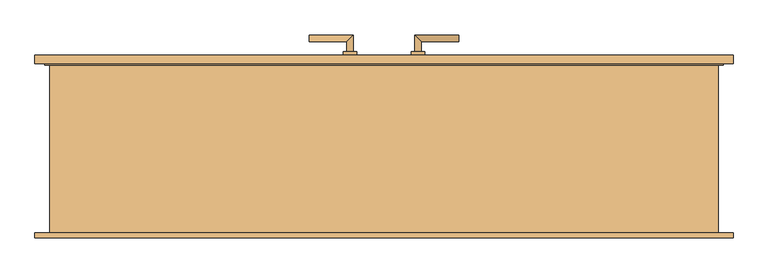
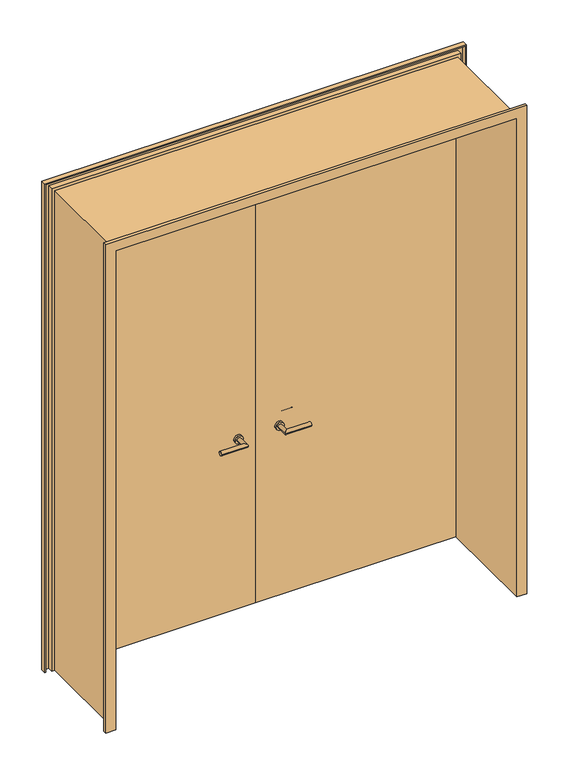
"""IFC4 building model written with IfcOpenShell, lengths in millimetres: door geometry, Drehflügel 2-flg - Variabel : Drehflügel 2-flg - Variabel."""

from ifc_helpers import new_model, si_unit, point, frame, frame_2d, origin, place, context, project, spatial, polyline, circle_curve, ellipse_curve, trimmed, segment, composite_curve, outline, extrude, faceted_brep, source, transform, mapped, element, save
from ifc_brep_helpers import plane_surface, cylinder_surface, advanced_brep


def door_c7457bb2(model_context):
    return source(origin(), model_context, "Body", "SolidModel", [
        advanced_brep(
        [(-90.0, 239.4346141, 1000.0), (-110.0, 239.4346141, 1000.0), (-110.0, 189.4346141, 1000.0), (-90.0, 169.4346141, 1000.0), (-220.0, 169.4346141, 1000.0), (-220.0, 189.4346141, 1000.0)],
        [
            (0, 1, circle_curve(frame((-100.0, 239.4346141, 1000.0), z_axis=(0.0, 1.0, 0.0), x_axis=(-1.0, 0.0, 0.0)), 10.0)),
            (1, 0, circle_curve(frame((-100.0, 239.4346141, 1000.0), z_axis=(0.0, 1.0, 0.0), x_axis=(-1.0, 0.0, 0.0)), 10.0)),
            (1, 2),
            (2, 3, ellipse_curve(frame((-100.0, 179.4346141, 1000.0), z_axis=(0.7071067811865385, 0.7071067811865565, 0.0), x_axis=(-0.7071067811865563, 0.7071067811865386, 0.0)), 14.1421356, 10.0)),
            (3, 0),
            (3, 2, ellipse_curve(frame((-100.0, 179.4346141, 1000.0), z_axis=(0.7071067811865385, 0.7071067811865565, 0.0), x_axis=(-0.7071067811865563, 0.7071067811865386, 0.0)), 14.1421356, 10.0)),
            (4, 5, circle_curve(frame((-220.0, 179.4346141, 1000.0), z_axis=(-1.0, 0.0, 0.0), x_axis=(0.0, 1.0, 0.0)), 10.0)),
            (5, 4, circle_curve(frame((-220.0, 179.4346141, 1000.0), z_axis=(-1.0, 0.0, 0.0), x_axis=(0.0, 1.0, 0.0)), 10.0)),
            (2, 5),
            (4, 3),
        ],
        [
            plane_surface(frame((-100.0, 239.4346141, -287.7526403), z_axis=(0.0, 1.0, 0.0), x_axis=(0.0, 0.0, 1.0))),
            cylinder_surface(frame((-100.0, 239.4346141, 1000.0), z_axis=(0.0, 1.0, 0.0), x_axis=(-1.0, 0.0, 0.0)), 10.0),
            plane_surface(frame((-220.0, 179.4346141, -287.7526403), z_axis=(-1.0, 0.0, 0.0), x_axis=(0.0, 0.0, 1.0))),
            cylinder_surface(frame((-100.0, 179.4346141, 1000.0), z_axis=(1.0, 0.0, 0.0), x_axis=(0.0, 1.0, 0.0)), 10.0),
        ],
        [
            (0, [[1, 2]]),
            (1, [[3, 4, 5, -2]]),
            (1, [[-5, 6, -3, -1]]),
            (2, [[7, 8]]),
            (3, [[9, -7, 10, -4]]),
            (3, [[-10, -8, -9, -6]]),
        ],
    ),
        advanced_brep(
        [(-110.0, 299.4346141, 1000.0), (-90.0, 299.4346141, 1000.0), (-90.0, 349.4346141, 1000.0), (-110.0, 329.4346141, 1000.0), (-220.0, 329.4346141, 1000.0), (-220.0, 349.4346141, 1000.0)],
        [
            (0, 1, circle_curve(frame((-100.0, 299.4346141, 1000.0), z_axis=(0.0, -1.0, 0.0), x_axis=(1.0, 0.0, 0.0)), 10.0)),
            (1, 0, circle_curve(frame((-100.0, 299.4346141, 1000.0), z_axis=(0.0, -1.0, 0.0), x_axis=(1.0, 0.0, 0.0)), 10.0)),
            (1, 2),
            (2, 3, ellipse_curve(frame((-100.0, 339.4346141, 1000.0), z_axis=(0.7071067811865475, -0.7071067811865475, 0.0), x_axis=(-0.7071067811865474, -0.7071067811865476, 0.0)), 14.1421356, 10.0)),
            (3, 0),
            (3, 2, ellipse_curve(frame((-100.0, 339.4346141, 1000.0), z_axis=(0.7071067811865475, -0.7071067811865475, 0.0), x_axis=(-0.7071067811865474, -0.7071067811865476, 0.0)), 14.1421356, 10.0)),
            (4, 5, circle_curve(frame((-220.0, 339.4346141, 1000.0), z_axis=(-1.0, 0.0, 0.0), x_axis=(0.0, 1.0, 0.0)), 10.0)),
            (5, 4, circle_curve(frame((-220.0, 339.4346141, 1000.0), z_axis=(-1.0, 0.0, 0.0), x_axis=(0.0, 1.0, 0.0)), 10.0)),
            (2, 5),
            (4, 3),
        ],
        [
            plane_surface(frame((-100.0, 299.4346141, -287.7526403), z_axis=(0.0, -1.0, 0.0), x_axis=(0.0, 0.0, 1.0))),
            cylinder_surface(frame((-100.0, 299.4346141, 1000.0), z_axis=(0.0, -1.0, 0.0), x_axis=(1.0, 0.0, 0.0)), 10.0),
            plane_surface(frame((-220.0, 339.4346141, -287.7526403), z_axis=(-1.0, 0.0, 0.0), x_axis=(0.0, 0.0, 1.0))),
            cylinder_surface(frame((-100.0, 339.4346141, 1000.0), z_axis=(1.0, 0.0, 0.0), x_axis=(0.0, 1.0, 0.0)), 10.0),
        ],
        [
            (0, [[1, 2]]),
            (1, [[3, 4, 5, -2]]),
            (1, [[-5, 6, -3, -1]]),
            (2, [[7, 8]]),
            (3, [[9, -7, 10, -4]]),
            (3, [[-10, -8, -9, -6]]),
        ],
    ),
        extrude(outline(composite_curve([segment(trimmed(circle_curve(frame_2d((1000.0, -100.0)), 20.0), [point((1000.0, -80.0))], [point((1000.0, -120.0))], False, "CARTESIAN"), True, "CONTINUOUS"), segment(trimmed(circle_curve(frame_2d((1000.0, -100.0)), 20.0), [point((1000.0, -120.0))], [point((1000.0, -80.0))], False, "CARTESIAN"), True, "CONTINUOUS")], self_intersect=False)), frame((0.0, 229.4346141, 0.0), z_axis=(0.0, 1.0, 0.0), x_axis=(0.0, 0.0, 1.0)), (0.0, 0.0, 1.0), 10.0),
        extrude(outline(composite_curve([segment(trimmed(circle_curve(frame_2d((1000.0, -100.0)), 20.0), [point((1000.0, -80.0))], [point((1000.0, -120.0))], False, "CARTESIAN"), True, "CONTINUOUS"), segment(trimmed(circle_curve(frame_2d((1000.0, -100.0)), 20.0), [point((1000.0, -120.0))], [point((1000.0, -80.0))], False, "CARTESIAN"), True, "CONTINUOUS")], self_intersect=False)), frame((0.0, 289.4346141, 0.0), z_axis=(0.0, 1.0, 0.0), x_axis=(0.0, 0.0, 1.0)), (0.0, 0.0, 1.0), 10.0),
        advanced_brep(
        [(90.0, 239.4346141, 1000.0), (110.0, 239.4346141, 1000.0), (90.0, 169.4346141, 1000.0), (110.0, 189.4346141, 1000.0), (220.0, 169.4346141, 1000.0), (220.0, 189.4346141, 1000.0)],
        [
            (0, 1, circle_curve(frame((100.0, 239.4346141, 1000.0), z_axis=(0.0, 1.0, 0.0), x_axis=(1.0, 0.0, 0.0)), 10.0)),
            (1, 0, circle_curve(frame((100.0, 239.4346141, 1000.0), z_axis=(0.0, 1.0, 0.0), x_axis=(1.0, 0.0, 0.0)), 10.0)),
            (0, 2),
            (2, 3, ellipse_curve(frame((100.0, 179.4346141, 1000.0), z_axis=(-0.7071067811865385, 0.7071067811865565, 0.0), x_axis=(0.7071067811865563, 0.7071067811865386, 0.0)), 14.1421356, 10.0)),
            (3, 1),
            (3, 2, ellipse_curve(frame((100.0, 179.4346141, 1000.0), z_axis=(-0.7071067811865385, 0.7071067811865565, 0.0), x_axis=(0.7071067811865563, 0.7071067811865386, 0.0)), 14.1421356, 10.0)),
            (4, 5, circle_curve(frame((220.0, 179.4346141, 1000.0), z_axis=(1.0, 0.0, 0.0), x_axis=(0.0, 1.0, 0.0)), 10.0)),
            (5, 4, circle_curve(frame((220.0, 179.4346141, 1000.0), z_axis=(1.0, 0.0, 0.0), x_axis=(0.0, 1.0, 0.0)), 10.0)),
            (2, 4),
            (5, 3),
        ],
        [
            plane_surface(frame((100.0, 239.4346141, -287.7526403), z_axis=(0.0, 1.0, 0.0), x_axis=(0.0, 0.0, 1.0))),
            cylinder_surface(frame((100.0, 239.4346141, 1000.0), z_axis=(0.0, 1.0, 0.0), x_axis=(1.0, 0.0, 0.0)), 10.0),
            plane_surface(frame((220.0, 179.4346141, -287.7526403), z_axis=(1.0, 0.0, 0.0), x_axis=(0.0, 0.0, 1.0))),
            cylinder_surface(frame((100.0, 179.4346141, 1000.0), z_axis=(-1.0, 0.0, 0.0), x_axis=(0.0, 1.0, 0.0)), 10.0),
        ],
        [
            (0, [[1, 2]]),
            (1, [[-1, 3, 4, 5]]),
            (1, [[-2, -5, 6, -3]]),
            (2, [[7, 8]]),
            (3, [[-4, 9, -8, 10]]),
            (3, [[-6, -10, -7, -9]]),
        ],
    ),
        advanced_brep(
        [(110.0, 299.4346141, 1000.0), (90.0, 299.4346141, 1000.0), (110.0, 329.4346141, 1000.0), (90.0, 349.4346141, 1000.0), (220.0, 329.4346141, 1000.0), (220.0, 349.4346141, 1000.0)],
        [
            (0, 1, circle_curve(frame((100.0, 299.4346141, 1000.0), z_axis=(0.0, -1.0, 0.0), x_axis=(-1.0, 0.0, 0.0)), 10.0)),
            (1, 0, circle_curve(frame((100.0, 299.4346141, 1000.0), z_axis=(0.0, -1.0, 0.0), x_axis=(-1.0, 0.0, 0.0)), 10.0)),
            (0, 2),
            (2, 3, ellipse_curve(frame((100.0, 339.4346141, 1000.0), z_axis=(-0.7071067811865475, -0.7071067811865475, 0.0), x_axis=(0.7071067811865474, -0.7071067811865476, 0.0)), 14.1421356, 10.0)),
            (3, 1),
            (3, 2, ellipse_curve(frame((100.0, 339.4346141, 1000.0), z_axis=(-0.7071067811865475, -0.7071067811865475, 0.0), x_axis=(0.7071067811865474, -0.7071067811865476, 0.0)), 14.1421356, 10.0)),
            (4, 5, circle_curve(frame((220.0, 339.4346141, 1000.0), z_axis=(1.0, 0.0, 0.0), x_axis=(0.0, 1.0, 0.0)), 10.0)),
            (5, 4, circle_curve(frame((220.0, 339.4346141, 1000.0), z_axis=(1.0, 0.0, 0.0), x_axis=(0.0, 1.0, 0.0)), 10.0)),
            (2, 4),
            (5, 3),
        ],
        [
            plane_surface(frame((100.0, 299.4346141, -287.7526403), z_axis=(0.0, -1.0, 0.0), x_axis=(0.0, 0.0, 1.0))),
            cylinder_surface(frame((100.0, 299.4346141, 1000.0), z_axis=(0.0, -1.0, 0.0), x_axis=(-1.0, 0.0, 0.0)), 10.0),
            plane_surface(frame((220.0, 339.4346141, -287.7526403), z_axis=(1.0, 0.0, 0.0), x_axis=(0.0, 0.0, 1.0))),
            cylinder_surface(frame((100.0, 339.4346141, 1000.0), z_axis=(-1.0, 0.0, 0.0), x_axis=(0.0, 1.0, 0.0)), 10.0),
        ],
        [
            (0, [[1, 2]]),
            (1, [[-1, 3, 4, 5]]),
            (1, [[-2, -5, 6, -3]]),
            (2, [[7, 8]]),
            (3, [[-4, 9, -8, 10]]),
            (3, [[-6, -10, -7, -9]]),
        ],
    ),
        extrude(outline(composite_curve([segment(trimmed(circle_curve(frame_2d((1000.0, 100.0)), 20.0), [point((1000.0, 80.0))], [point((1000.0, 120.0))], False, "CARTESIAN"), True, "CONTINUOUS"), segment(trimmed(circle_curve(frame_2d((1000.0, 100.0)), 20.0), [point((1000.0, 120.0))], [point((1000.0, 80.0))], False, "CARTESIAN"), True, "CONTINUOUS")], self_intersect=False)), frame((0.0, 229.4346141, 0.0), z_axis=(0.0, 1.0, 0.0), x_axis=(0.0, 0.0, 1.0)), (0.0, 0.0, 1.0), 10.0),
        extrude(outline(composite_curve([segment(trimmed(circle_curve(frame_2d((1000.0, 100.0)), 20.0), [point((1000.0, 80.0))], [point((1000.0, 120.0))], False, "CARTESIAN"), True, "CONTINUOUS"), segment(trimmed(circle_curve(frame_2d((1000.0, 100.0)), 20.0), [point((1000.0, 120.0))], [point((1000.0, 80.0))], False, "CARTESIAN"), True, "CONTINUOUS")], self_intersect=False)), frame((0.0, 289.4346141, 0.0), z_axis=(0.0, 1.0, 0.0), x_axis=(0.0, 0.0, 1.0)), (0.0, 0.0, 1.0), 10.0),
        extrude(outline(polyline([(0.0, 264.4346141), (-995.0, 264.4346141), (-995.0, 289.4346141), (0.0, 289.4346141), (0.0, 264.4346141)])), frame((0.0, 0.0, 100.0), z_axis=(0.0, 0.0, 1.0), x_axis=(1.0, 0.0, 0.0)), (0.0, 0.0, 1.0), 2490.0),
        extrude(outline(polyline([(995.0, 264.4346141), (0.0, 264.4346141), (0.0, 289.4346141), (995.0, 289.4346141), (995.0, 264.4346141)])), frame((0.0, 0.0, 100.0), z_axis=(0.0, 0.0, 1.0), x_axis=(1.0, 0.0, 0.0)), (0.0, 0.0, 1.0), 2490.0),
        faceted_brep([(1029.5, -250.5653859, 100.0), (980.0, -250.5653859, 100.0), (980.0, 264.4346141, 100.0), (995.0, 264.4346141, 100.0), (995.0, 289.4346141, 100.0), (1029.5, 289.4346141, 100.0), (1029.5, 264.4346141, 100.0), (1024.5, 264.4346141, 100.0), (1024.5, 284.4346141, 100.0), (1000.0, 284.4346141, 100.0), (1000.0, 259.4346141, 100.0), (985.0, 259.4346141, 100.0), (985.0, -245.5653859, 100.0), (1024.5, -245.5653859, 100.0), (1024.5, -235.5653859, 100.0), (1029.5, -235.5653859, 100.0), (1029.5, -250.5653859, 2624.5), (-1029.5, -250.5653859, 2624.5), (-1029.5, -250.5653859, 100.0), (-980.0, -250.5653859, 100.0), (-980.0, -250.5653859, 2575.0), (980.0, -250.5653859, 2575.0), (980.0, 264.4346141, 2575.0), (-980.0, 264.4346141, 2575.0), (-980.0, 264.4346141, 100.0), (-995.0, 264.4346141, 100.0), (-995.0, 264.4346141, 2590.0), (995.0, 264.4346141, 2590.0), (995.0, 289.4346141, 2590.0), (-995.0, 289.4346141, 2590.0), (-995.0, 289.4346141, 100.0), (-1029.5, 289.4346141, 100.0), (-1029.5, 289.4346141, 2624.5), (1029.5, 289.4346141, 2624.5), (1029.5, 264.4346141, 2624.5), (-1029.5, 264.4346141, 2624.5), (-1029.5, 264.4346141, 100.0), (-1024.5, 264.4346141, 100.0), (-1024.5, 264.4346141, 2619.5), (1024.5, 264.4346141, 2619.5), (1024.5, 284.4346141, 2619.5), (-1024.5, 284.4346141, 2619.5), (-1024.5, 284.4346141, 100.0), (-1000.0, 284.4346141, 100.0), (-1000.0, 284.4346141, 2595.0), (1000.0, 284.4346141, 2595.0), (1000.0, 259.4346141, 2595.0), (-1000.0, 259.4346141, 2595.0), (-1000.0, 259.4346141, 100.0), (-985.0, 259.4346141, 100.0), (-985.0, 259.4346141, 2580.0), (985.0, 259.4346141, 2580.0), (985.0, -245.5653859, 2580.0), (-985.0, -245.5653859, 2580.0), (-985.0, -245.5653859, 100.0), (-1024.5, -245.5653859, 100.0), (-1024.5, -245.5653859, 2619.5), (1024.5, -245.5653859, 2619.5), (1024.5, -235.5653859, 2619.5), (-1024.5, -235.5653859, 2619.5), (-1024.5, -235.5653859, 100.0), (-1029.5, -235.5653859, 100.0), (-1029.5, -235.5653859, 2624.5), (1029.5, -235.5653859, 2624.5)], [[[0, 1, 2, 3, 4, 5, 6, 7, 8, 9, 10, 11, 12, 13, 14, 15]], [[1, 0, 16, 17, 18, 19, 20, 21]], [[2, 1, 21, 22]], [[3, 2, 22, 23, 24, 25, 26, 27]], [[4, 3, 27, 28]], [[5, 4, 28, 29, 30, 31, 32, 33]], [[6, 5, 33, 34]], [[7, 6, 34, 35, 36, 37, 38, 39]], [[8, 7, 39, 40]], [[9, 8, 40, 41, 42, 43, 44, 45]], [[10, 9, 45, 46]], [[11, 10, 46, 47, 48, 49, 50, 51]], [[12, 11, 51, 52]], [[13, 12, 52, 53, 54, 55, 56, 57]], [[14, 13, 57, 58]], [[15, 14, 58, 59, 60, 61, 62, 63]], [[0, 15, 63, 16]], [[17, 62, 61, 18]], [[18, 61, 60, 55, 54, 49, 48, 43, 42, 37, 36, 31, 30, 25, 24, 19]], [[23, 20, 19, 24]], [[29, 26, 25, 30]], [[35, 32, 31, 36]], [[41, 38, 37, 42]], [[47, 44, 43, 48]], [[53, 50, 49, 54]], [[59, 56, 55, 60]], [[22, 21, 20, 23]], [[28, 27, 26, 29]], [[34, 33, 32, 35]], [[40, 39, 38, 41]], [[46, 45, 44, 47]], [[52, 51, 50, 53]], [[58, 57, 56, 59]], [[16, 63, 62, 17]]]),
    ])


if __name__ == "__main__":
    model = new_model("IFC4")
    model_context = context("Model", 3, world=origin())
    ifc_project = project(units=[si_unit("LENGTHUNIT", "METRE", prefix="MILLI")], contexts=[model_context])
    site = spatial("IfcSite", under=ifc_project)
    building = spatial("IfcBuilding", under=site)
    placement = place(None, origin())
    door_shape = door_c7457bb2(model_context)
    element("IfcDoor", 1, ObjectType="Drehflügel 2-flg - Variabel : Drehflügel 2-flg - Variabel", at=placement, inside=building, context=model_context, shape_type="MappedRepresentation", body=[
        mapped(door_shape, transform((0.0, 0.0, 0.0), x_axis=(1.0, 0.0, 0.0), y_axis=(0.0, 1.0, 0.0), z_axis=(0.0, 0.0, 1.0))),
    ])
    save(model, "model.ifc")

# Revit data of these elements
# Type "Drehflügel 2-flg - Variabel : Drehflügel 2-flg - Variabel"
#   Construction Type Id = "MDOOR"
#   Type Mark = "18"
#   Operation = "DoubleDoorSingleSwing"
#   Keynote = "16.03"
#   Analytic Construction = "Metall"
#   Thermal Resistance (R) = 0.270117 (m²·K)/W
#   Heat Transfer Coefficient (U) = 3.7021 W/(m²·K)
#   Rough Width [instance default] = 2.010 m
#   Rough Height [instance default] = 2.360 m
#   Höhe Türgriff = 0.900 m
#   Height [instance default] = 2.260 m
#   Fußbodenaufbau [instance default] = 0.100 m
#   Width [instance default] = 2.010 m
#   Sichtbarkeit Sturzlinien [instance default] = yes
#   Türgriff auswählen [instance default] = element 222671
#   Türgriff [instance default] = none
#   Türflügel [instance default] = none
#   Rahmen/Pfosten [instance default] = Metall - Lackiert - Grau
#   Visual Light Transmittance = 0
#   Solar Heat Gain Coefficient = 0
#   Function = (empty or 0)
#   Wall Closure = (empty or 0)
# Element 1 (IfcDoor, "Drehflügel 2-flg - Variabel : Drehflügel 2-flg - Variabel")
#   Rough Height = 2.600 m
#   Height = 2.500 m
#   Materials on its faces: "Metall - Chrom", "Metall - Lackiert - Grau", "Holz - Birke"
# Materials
#   "Metall - Lackiert - Grau": class "Farbe 1", colour RGB 98 98 98, transparency 0, Cost = 0
#   "Metall - Chrom": class "Metall", colour RGB 247 247 247, transparency 0, Cost = 0
#   "Holz - Birke": class "Holz", colour RGB 213 164 103, transparency 0, Cost = 0
